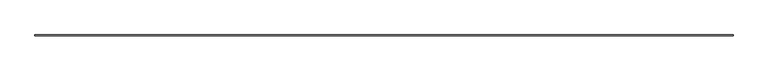
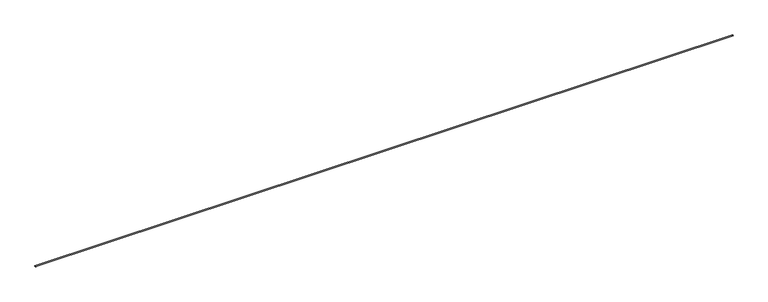
"""IFC4 building model written with IfcOpenShell, lengths in millimetres: proxy geometry, Inner panel:Inner panel:1:Inner panel:1 : Inner panel:Inner panel:300324:2:Inner panel:1:Inner panel:1 : Inner panel:Inner panel:300324:2 : Inner panel:Inner panel:1:Inner panel:1 : Inner panel:Inner panel:300324:300043:24 : Inner panel:Inner panel:1:Inner panel:1 : Inner panel:Inner panel:300324:2:Inner panel:1:Inner panel:1 : Inner panel:Inner panel:300324:2 : Inner panel:Inner panel:1:Inner panel:1 : Inner panel:Inner panel:300324:300043:308120."""

from ifc_helpers import new_model, si_unit, frame, origin, place, context, project, spatial, polyline, outline, extrude, source, transform, mapped, element, save


def generic_models_f21c0271(model_context):
    return source(origin(), model_context, "Body", "SweptSolid", [
        extrude(outline(polyline([(0.0, -25.3999999), (0.0, 0.0), (17694.2750003, 0.0), (17694.2750003, -25.3999999), (0.0, -25.3999999)])), frame((596798.7867242, -579086.4260178, 3946.326075), z_axis=(0.0, -0.0416305447122168, 0.9991330730923504), x_axis=(-1.0, 0.0, 0.0)), (0.0, 0.0, 1.0), 9.525),
    ])


if __name__ == "__main__":
    model = new_model("IFC4")
    model_context = context("Model", 3, world=origin())
    ifc_project = project(units=[si_unit("LENGTHUNIT", "METRE", prefix="MILLI")], contexts=[model_context])
    site = spatial("IfcSite", under=ifc_project)
    building = spatial("IfcBuilding", under=site)
    placement = place(None, origin())
    generic_models_shape = generic_models_f21c0271(model_context)
    element("IfcBuildingElementProxy", 1, Name="Inner panel:Inner panel:1:Inner panel:1 : Inner panel:Inner panel:300324:2:Inner panel:1:Inner panel:1 : Inner panel:Inner panel:300324:2 : Inner panel:Inner panel:1:Inner panel:1 : Inner panel:Inner panel:300324:300043:24 : Inner panel:Inner panel:1:Inner panel:1 : Inner panel:Inner panel:300324:2:Inner panel:1:Inner panel:1 : Inner panel:Inner panel:300324:2 : Inner panel:Inner panel:1:Inner panel:1 : Inner panel:Inner panel:300324:300043:308120", ObjectType="Inner panel:Inner panel:1:Inner panel:1 : Inner panel:Inner panel:300324:2:Inner panel:1:Inner panel:1 : Inner panel:Inner panel:300324:2 : Inner panel:Inner panel:1:Inner panel:1 : Inner panel:Inner panel:300324:300043:24 : Inner panel:Inner panel:1:Inner panel:1 : Inner panel:Inner panel:300324:2:Inner panel:1:Inner panel:1 : Inner panel:Inner panel:300324:2 : Inner panel:Inner panel:1:Inner panel:1 : Inner panel:Inner panel:300324:300043:308120", at=placement, inside=building, context=model_context, shape_type="MappedRepresentation", body=[
        mapped(generic_models_shape, transform((0.0, 0.0, 0.0), x_axis=(1.0, 0.0, 0.0), y_axis=(0.0, 1.0, 0.0), z_axis=(0.0, 0.0, 1.0))),
    ])
    save(model, "model.ifc")

# Revit data of these elements
# Type "Inner panel:Inner panel:1:Inner panel:1 : Inner panel:Inner panel:300324:2:Inner panel:1:Inner panel:1 : Inner panel:Inner panel:300324:2 : Inner panel:Inner panel:1:Inner panel:1 : Inner panel:Inner panel:300324:300043:24 : Inner panel:Inner panel:1:Inner panel:1 : Inner panel:Inner panel:300324:2:Inner panel:1:Inner panel:1 : Inner panel:Inner panel:300324:2 : Inner panel:Inner panel:1:Inner panel:1 : Inner panel:Inner panel:300324:300043:308120"
#   NameOverride = "Inner panel:Inner panel:1:Inner panel:1 : Inner panel:Inner panel:300324:2:Inner panel:1:Inner panel:1 : Inner panel:Inner panel:300324:2 : Inner panel:Inner panel:1:Inner panel:1 : Inner panel:Inner panel:300324:300043:308120"
#   ObjectTypeOverride = "Inner panel:1:Inner panel:1 : Inner panel:Inner panel:300324:2 : Inner panel:Inner panel:1:Inner panel:1 : Inner panel:Inner panel:300324:300043"
#   Reference = "Inner panel"
#   Tag = "308120"
# Element 1 (IfcBuildingElementProxy, "Inner panel:Inner panel:1:Inner panel:1 : Inner panel:Inner panel:300324:2:Inner panel:1:Inner panel:1 : Inner panel:Inner panel:300324:2 : Inner panel:Inner panel:1:Inner panel:1 : Inner panel:Inner panel:300324:300043:24 : Inner panel:Inner panel:1:Inner panel:1 : Inner panel:Inner panel:300324:2:Inner panel:1:Inner panel:1 : Inner panel:Inner panel:300324:2 : Inner panel:Inner panel:1:Inner panel:1 : Inner panel:Inner panel:300324:300043:308120")
#   Materials on its faces: "1\" WIDE NON ABSORBENT, COMPRESSIBLE, WEATHER-RESISTANT NEOPRENE/EPDM/SBR FOAM (25% THICKER THAN GAP)"
# Materials
#   "1\" WIDE NON ABSORBENT, COMPRESSIBLE, WEATHER-RESISTANT NEOPRENE/EPDM/SBR FOAM (25% THICKER THAN GAP)": class "Generic", colour RGB 120 120 120, transparency 0, Cost = 0
